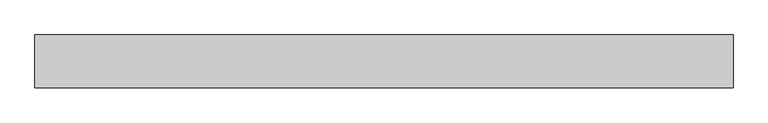
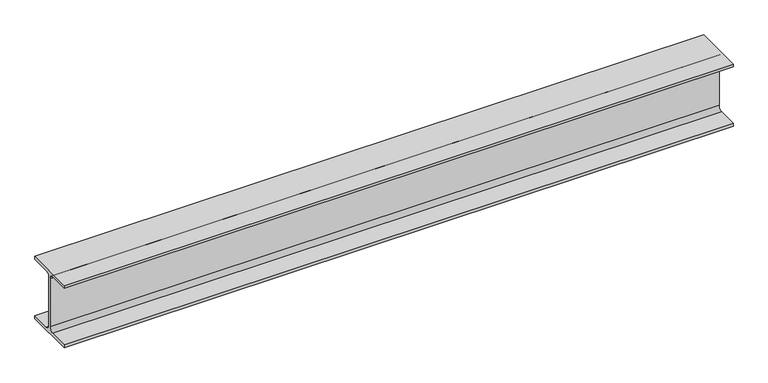
"""IFC4 building model written with IfcOpenShell, lengths in millimetres: beam geometry, 0912_Steel Framing_H-KSD3502 : H_SB_ASB_H-194x150x6x9."""

from ifc_helpers import new_model, si_unit, point, frame, frame_2d, origin, place, context, project, spatial, polyline, circle_curve, trimmed, segment, composite_curve, outline, extrude, source, transform, mapped, element, save


def beam_60b30bf3(model_context):
    return source(origin(), model_context, "Body", "SweptSolid", [
        extrude(outline(composite_curve([segment(polyline([(-75.0, -88.0), (-16.0, -88.0)]), True, "CONTINUOUS"), segment(trimmed(circle_curve(frame_2d((-16.0, -75.0)), 13.0), [point((-16.0, -88.0))], [point((-3.0, -75.0))], True, "CARTESIAN"), True, "CONTINUOUS"), segment(polyline([(-3.0, -75.0), (-3.0, 75.0)]), True, "CONTINUOUS"), segment(trimmed(circle_curve(frame_2d((-16.0, 75.0)), 13.0), [point((-3.0, 75.0))], [point((-16.0, 88.0))], True, "CARTESIAN"), True, "CONTINUOUS"), segment(polyline([(-16.0, 88.0), (-75.0, 88.0), (-75.0, 97.0), (75.0, 97.0), (75.0, 88.0), (16.0, 88.0)]), True, "CONTINUOUS"), segment(trimmed(circle_curve(frame_2d((16.0, 75.0)), 13.0), [point((16.0, 88.0))], [point((3.0, 75.0))], True, "CARTESIAN"), True, "CONTINUOUS"), segment(polyline([(3.0, 75.0), (3.0, -75.0)]), True, "CONTINUOUS"), segment(trimmed(circle_curve(frame_2d((16.0, -75.0)), 13.0), [point((3.0, -75.0))], [point((16.0, -88.0))], True, "CARTESIAN"), True, "CONTINUOUS"), segment(polyline([(16.0, -88.0), (75.0, -88.0), (75.0, -97.0), (-75.0, -97.0), (-75.0, -88.0)]), True, "CONTINUOUS")], self_intersect=False)), frame((-988.3546085, 0.0, 0.0), z_axis=(1.0, 0.0, 0.0), x_axis=(0.0, 1.0, 0.0)), (0.0, 0.0, 1.0), 1976.709217),
    ])


if __name__ == "__main__":
    model = new_model("IFC4")
    model_context = context("Model", 3, world=origin())
    ifc_project = project(units=[si_unit("LENGTHUNIT", "METRE", prefix="MILLI")], contexts=[model_context])
    site = spatial("IfcSite", under=ifc_project)
    building = spatial("IfcBuilding", under=site)
    placement = place(None, origin())
    beam_shape = beam_60b30bf3(model_context)
    element("IfcBeam", 1, ObjectType="0912_Steel Framing_H-KSD3502 : H_SB_ASB_H-194x150x6x9", at=placement, inside=building, context=model_context, shape_type="MappedRepresentation", body=[
        mapped(beam_shape, transform((0.0, 0.0, 0.0), x_axis=(1.0, 0.0, 0.0), y_axis=(0.0, 1.0, 0.0), z_axis=(0.0, 0.0, 1.0))),
    ])
    save(model, "model.ifc")

# Revit data of these elements
# Type "0912_Steel Framing_H-KSD3502 : H_SB_ASB_H-194x150x6x9"
#   H_WM Code_1 = "S01AA002-00001 | Main Steel Structure Fabrication Work | Shelter/Building | Medium Steel - Standard (90KG/M>Weight≥30KG/M) | Material: (   )"
#   H_WM Code_2 = "S03AA028-00001 | Main Steel Structure Erection Work | Shelter/Building | Medium Steel (90KG/M>Weight≥30KG/M) | Material: (   )"
#   H_WM Code_3 = "S01AA010-00001 | Main Steel Structure Fabrication Work | Shelter/Building | Steel Painting/Coating | for Non-Fireproofed Steel Surface, Surface Preparation, Primer, Second & Final Coat | Material: (   )"
#   H_Q'ty Cal Type Tag = "SB-Q2"
#   Width = 15.0 cm
#   Web Thickness = 0.6 cm
#   Web Fillet = 1.3 cm
#   Warping Constant = 43316.0 cm⁶
#   W = 0
#   Torsional Moment of Inertia = 8.622 cm⁴
#   Section Area = 39.01 cm²
#   Plastic Modulus weak axis = 104.0 cm³
#   Plastic Modulus strong axis = 309.0 cm³
#   Perimeter = 0.95 m²/m
#   Nominal Weight = 30.60 kgf/m
#   Moment of Inertia weak axis = 507.00 cm⁴
#   Moment of Inertia strong axis = 2690.00 cm⁴
#   Height = 19.4 cm
#   Flange Thickness = 0.9 cm
#   Elastic Modulus weak axis = 67.6 cm³
#   Elastic Modulus strong axis = 277.0 cm³
#   Centroid Vertical = 9.7 cm
#   Centroid Horizontal = 7.5 cm
#   Ix = 26900000
#   Length [instance default] = 1.5240 m
#   Zx = 309000
#   b = 0.1500 m
#   h = 0.1940 m
#   r = 0.0130 m
#   s = 0.0060 m
#   t = 0.0090 m
#   A = 0.003901 m²
#   Structural Material [instance default] = Steel, 45-345
#   Assembly Code = ""
# Element 1 (IfcBeam, "0912_Steel Framing_H-KSD3502 : H_SB_ASB_H-194x150x6x9")
#   Structural Material = none
# Materials
#   "Steel, 45-345": class "Metal", colour RGB 189 187 185, transparency 0, Description = "Steel 345 MPa", Cost = 0
